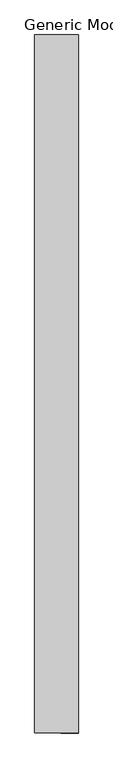
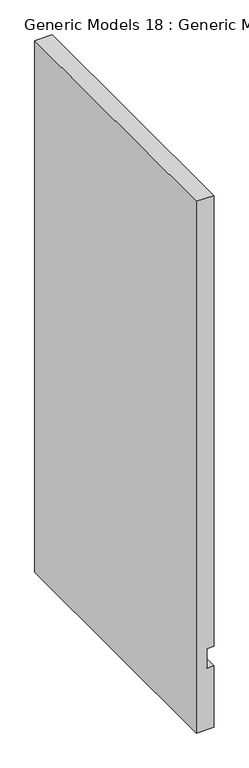
"""IFC4 building model written with IfcOpenShell, lengths in millimetres: proxy geometry, Generic Models 18 : Generic Models 1."""

from ifc_helpers import new_model, si_unit, frame, origin, place, context, project, spatial, polyline, outline, extrude, source, transform, mapped, element, save


def generic_models_18_generic_models_1_46f1d7c3(model_context):
    return source(origin(), model_context, "Body", "SweptSolid", [
        extrude(outline(polyline([(-1916.5098206, 52566.3071108), (-1916.5098206, 52642.5071108), (-1633.3277575, 52642.5071108), (-1633.3277575, 52612.3446108), (-1544.4277575, 52612.3446108), (-1544.4277575, 52642.5071108), (528.2401794, 52642.5071108), (528.2401794, 52566.3071108), (-1916.5098206, 52566.3071108)])), frame((0.0, 0.0, 0.0), z_axis=(0.0, 1.0, 0.0), x_axis=(0.0, 0.0, 1.0)), (0.0, 0.0, 1.0), 1219.2),
    ])


if __name__ == "__main__":
    model = new_model("IFC4")
    model_context = context("Model", 3, world=origin())
    ifc_project = project(units=[si_unit("LENGTHUNIT", "METRE", prefix="MILLI")], contexts=[model_context])
    site = spatial("IfcSite", under=ifc_project)
    building = spatial("IfcBuilding", under=site)
    placement = place(None, origin())
    generic_models_18_generic_models_1_shape = generic_models_18_generic_models_1_46f1d7c3(model_context)
    element("IfcBuildingElementProxy", 1, Name="Generic Models 18 : Generic Models 1", ObjectType="Generic Models 18 : Generic Models 1", at=placement, inside=building, context=model_context, shape_type="MappedRepresentation", body=[
        mapped(generic_models_18_generic_models_1_shape, transform((0.0, 0.0, 0.0), x_axis=(1.0, 0.0, 0.0), y_axis=(0.0, 1.0, 0.0), z_axis=(0.0, 0.0, 1.0))),
    ])
    save(model, "model.ifc")

# Revit data of these elements
# Element 1 (IfcBuildingElementProxy, "Generic Models 18 : Generic Models 1")
#   Materials on its faces: "(S) SOUND BATT. INSULATION (THICKNESS TO MATCH WALL DEPTH)"
# Materials
#   "(S) SOUND BATT. INSULATION (THICKNESS TO MATCH WALL DEPTH)": class "Unassigned", colour RGB 255 255 255, transparency 0, Cost = 0
